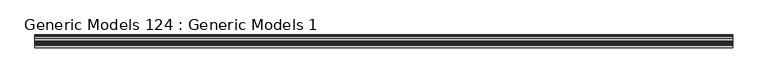
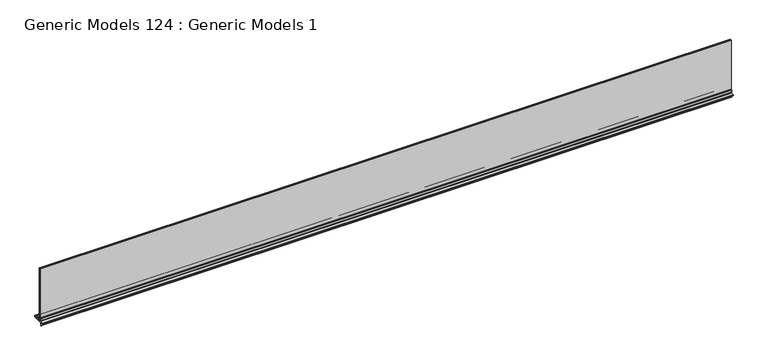
"""IFC4 building model written with IfcOpenShell, lengths in millimetres: proxy geometry, Generic Models 124 : Generic Models 1."""

import ifcopenshell
import ifcopenshell.guid

model = None  # the IFC model being written
_history = None  # IfcOwnerHistory: only IFC2X3 demands one
_inside = {}  # id of a spatial element -> (the spatial element, [elements in it])
_under = {}  # id of a project, library or spatial element -> (it, [spatial elements below it])
_declared = {}  # id of a project -> (the project, [libraries it declares])
_typed = {}  # id of a type object -> (the type object, [elements of that type])
_made_of = {}  # id of a material, layer set ... -> (it, [elements and type objects made of it])


def new_model(schema):
    """Start an empty IFC model of exactly this schema.

    Asked for "IFC4X3", IfcOpenShell would pick the latest addendum, in which some entities
    have other attributes; the version numbers below select the first issue.
    IFC2X3 requires an IfcOwnerHistory on every rooted entity: one is made here for all.
    """
    global model, _history
    if schema == "IFC4X3":
        model = ifcopenshell.file(schema_version=(4, 3, 0, 0))
    else:
        model = ifcopenshell.file(schema=schema)
    _inside.clear()
    _under.clear()
    _declared.clear()
    _typed.clear()
    _made_of.clear()
    _history = None
    if model.schema == "IFC2X3":
        org = make("IfcOrganization", Name="unknown")
        user = make(
            "IfcPersonAndOrganization",
            ThePerson=make("IfcPerson", FamilyName="unknown"),
            TheOrganization=org,
        )
        app = make(
            "IfcApplication",
            ApplicationDeveloper=org,
            Version="unknown",
            ApplicationFullName="unknown",
            ApplicationIdentifier="unknown",
        )
        _history = make(
            "IfcOwnerHistory",
            OwningUser=user,
            OwningApplication=app,
            ChangeAction="ADDED",
            CreationDate=0,
        )
    return model


def make(cls, **values):
    """One entity of the class cls with the attributes given. An attribute that is None is left unset."""
    return model.create_entity(
        cls, **{name: value for name, value in values.items() if value is not None}
    )


def rooted(cls, **values):
    """An entity with a GlobalId (a new one), such as an element, a storey or a relation."""
    return make(cls, GlobalId=ifcopenshell.guid.new(), OwnerHistory=_history, **values)


def si_unit(unit_type, name, prefix=None):
    """IfcSIUnit, for example si_unit("LENGTHUNIT", "METRE", prefix="MILLI")."""
    return make("IfcSIUnit", UnitType=unit_type, Prefix=prefix, Name=name)


def assignment(units):
    """IfcUnitAssignment: the units of a project."""
    return None if units is None else make("IfcUnitAssignment", Units=units)


def point(xyz):
    """IfcCartesianPoint."""
    return None if xyz is None else make("IfcCartesianPoint", Coordinates=xyz)


def direction(xyz):
    """IfcDirection."""
    return None if xyz is None else make("IfcDirection", DirectionRatios=xyz)


def frame(location, z_axis=None, x_axis=None):
    """IfcAxis2Placement3D, a coordinate frame: its origin and axes. An axis left out is left unset."""
    return make(
        "IfcAxis2Placement3D",
        Location=point(location),
        Axis=direction(z_axis),
        RefDirection=direction(x_axis),
    )


def frame_2d(location, x_axis=None):
    """IfcAxis2Placement2D, a coordinate frame in the plane: its origin and x axis."""
    return make(
        "IfcAxis2Placement2D", Location=point(location), RefDirection=direction(x_axis)
    )


def origin():
    """The frame at (0, 0, 0) with its axes left unset."""
    return frame((0.0, 0.0, 0.0))


def place(relative_to, where):
    """IfcLocalPlacement: puts the frame where relative to a parent placement (None: the world)."""
    return make(
        "IfcLocalPlacement", PlacementRelTo=relative_to, RelativePlacement=where
    )


def context(
    kind, dimensions, precision=None, world=None, true_north=None, identifier=None
):
    """IfcGeometricRepresentationContext, for example the 3D "Model" context."""
    return make(
        "IfcGeometricRepresentationContext",
        ContextIdentifier=identifier,
        ContextType=kind,
        CoordinateSpaceDimension=dimensions,
        Precision=precision,
        WorldCoordinateSystem=world,
        TrueNorth=true_north,
    )


def project(units=None, contexts=None):
    """IfcProject with its units and contexts."""
    return rooted(
        "IfcProject",
        Name="project",
        RepresentationContexts=contexts,
        UnitsInContext=assignment(units),
    )


def spatial(cls, under=None, at=None, **own):
    """A site, building, storey or space (cls), placed at a placement, below another one or the project."""
    s = rooted(cls, ObjectPlacement=at, **own)
    if under is not None:
        _under.setdefault(under.id(), (under, []))[1].append(s)
    return s


def polyline(points):
    """IfcPolyline through the points."""
    return make("IfcPolyline", Points=[point(p) for p in points])


def circle_curve(where, radius):
    """IfcCircle in the frame where."""
    return make("IfcCircle", Position=where, Radius=radius)


def trimmed(basis, trim1, trim2, sense, master):
    """IfcTrimmedCurve: the piece of a basis curve between two trims."""
    return make(
        "IfcTrimmedCurve",
        BasisCurve=basis,
        Trim1=trim1,
        Trim2=trim2,
        SenseAgreement=sense,
        MasterRepresentation=master,
    )


def segment(curve, same_sense, transition):
    """IfcCompositeCurveSegment."""
    return make(
        "IfcCompositeCurveSegment",
        Transition=transition,
        SameSense=same_sense,
        ParentCurve=curve,
    )


def composite_curve(segments, self_intersect=None):
    """IfcCompositeCurve: segments joined end to end."""
    return make("IfcCompositeCurve", Segments=segments, SelfIntersect=self_intersect)


def outline(outer, holes=None, kind="AREA"):
    """IfcArbitraryClosedProfileDef: a profile drawn as a closed curve; with holes, ...WithVoids."""
    if holes is None:
        return make("IfcArbitraryClosedProfileDef", ProfileType=kind, OuterCurve=outer)
    return make(
        "IfcArbitraryProfileDefWithVoids",
        ProfileType=kind,
        OuterCurve=outer,
        InnerCurves=holes,
    )


def extrude(swept, where, along, depth):
    """IfcExtrudedAreaSolid: the profile swept, set in the frame where, extruded along a direction by depth."""
    return make(
        "IfcExtrudedAreaSolid",
        SweptArea=swept,
        Position=where,
        ExtrudedDirection=direction(along),
        Depth=depth,
    )


def shape(context_of_items, identifier, shape_type, items):
    """IfcShapeRepresentation: the items that make up one representation, for example the "Body"."""
    return make(
        "IfcShapeRepresentation",
        ContextOfItems=context_of_items,
        RepresentationIdentifier=identifier,
        RepresentationType=shape_type,
        Items=items,
    )


def source(mapping_origin, context_of_items, identifier, shape_type, items):
    """IfcRepresentationMap: a shape defined once, which mapped items show again and again."""
    return make(
        "IfcRepresentationMap",
        MappingOrigin=mapping_origin,
        MappedRepresentation=shape(context_of_items, identifier, shape_type, items),
    )


def transform(
    local_origin,
    x_axis=None,
    y_axis=None,
    z_axis=None,
    scale=None,
    scale2=None,
    scale3=None,
    uniform=True,
):
    """IfcCartesianTransformationOperator3D, or its non-uniform kind. x_axis, y_axis, z_axis: its Axis1, 2, 3."""
    if uniform:
        return make(
            "IfcCartesianTransformationOperator3D",
            Axis1=direction(x_axis),
            Axis2=direction(y_axis),
            LocalOrigin=point(local_origin),
            Scale=scale,
            Axis3=direction(z_axis),
        )
    return make(
        "IfcCartesianTransformationOperator3DnonUniform",
        Axis1=direction(x_axis),
        Axis2=direction(y_axis),
        LocalOrigin=point(local_origin),
        Scale=scale,
        Axis3=direction(z_axis),
        Scale2=scale2,
        Scale3=scale3,
    )


def mapped(mapping_source, mapping_target):
    """IfcMappedItem: shows the shape of a source again, moved by a transform."""
    return make(
        "IfcMappedItem", MappingSource=mapping_source, MappingTarget=mapping_target
    )


def made_of(thing, what):
    """Note that an element or type object is made of a material, layer set ...; save() writes the relation."""
    if what is not None:
        _made_of.setdefault(what.id(), (what, []))[1].append(thing)
    return thing


def element(
    cls,
    number,
    at=None,
    inside=None,
    cuts=None,
    type_object=None,
    material=None,
    context=None,
    identifier="Body",
    shape_type=None,
    held_by="IfcProductDefinitionShape",
    body=None,
    shapes=None,
    **own,
):
    """One element of the class cls, such as IfcWall. Its Tag is "e" and its number.

    at: its placement. inside: the storey or other place that contains it. cuts: it is an
    opening in that element (IfcRelVoidsElement). A single representation is given by context,
    identifier, shape_type and body (its items); several are given by shapes. held_by: the class
    of the entity that holds the representations. save() writes the other relations.
    """
    e = rooted(cls, Tag="e%d" % number, ObjectPlacement=at, **own)
    if body is not None:
        shapes = [shape(context, identifier, shape_type, body)]
    if shapes is not None:
        e.Representation = make(held_by, Representations=shapes)
    if inside is not None:
        _inside.setdefault(inside.id(), (inside, []))[1].append(e)
    if cuts is not None:
        rooted(
            "IfcRelVoidsElement", RelatingBuildingElement=cuts, RelatedOpeningElement=e
        )
    if type_object is not None:
        _typed.setdefault(type_object.id(), (type_object, []))[1].append(e)
    return made_of(e, material)


def aggregate(whole, parts):
    """IfcRelAggregates: a whole, such as a stair, and the parts it consists of."""
    return rooted("IfcRelAggregates", RelatingObject=whole, RelatedObjects=parts)


def save(model, path):
    """Write the relations noted so far, then the file.

    IfcRelAggregates (storeys below a building ...), IfcRelContainedInSpatialStructure (elements
    in a storey), IfcRelDefinesByType, IfcRelAssociatesMaterial and IfcRelDeclares: one each for
    every whole, place, type object, material and project.
    """
    for whole, parts in _under.values():
        aggregate(whole, parts)
    for where, things in _inside.values():
        rooted(
            "IfcRelContainedInSpatialStructure",
            RelatedElements=things,
            RelatingStructure=where,
        )
    for kind, things in _typed.values():
        rooted("IfcRelDefinesByType", RelatedObjects=things, RelatingType=kind)
    for what, things in _made_of.values():
        rooted("IfcRelAssociatesMaterial", RelatedObjects=things, RelatingMaterial=what)
    for by, libraries in _declared.values():
        rooted("IfcRelDeclares", RelatingContext=by, RelatedDefinitions=libraries)
    model.write(path)


def generic_models_124_generic_models_1_1996d743(model_context):
    return source(origin(), model_context, "Body", "SweptSolid", [
        extrude(outline(composite_curve([segment(polyline([(6990.9493503, 124213.5950923), (6972.8808069, 124213.5950923), (6972.8808069, 124216.7700923), (6970.594803, 124216.7700923), (6970.594803, 124213.5950923), (6953.0870538, 124213.5950923), (6953.0870538, 124216.7700923), (6950.8010499, 124216.7700923), (6950.8010499, 124213.5950923), (6933.7739503, 124213.5950923), (6933.7739503, 124215.6778923), (6930.5989503, 124215.6778923), (6930.5989503, 124213.5950923), (6913.4995677, 124213.5950923), (6913.4995677, 124216.7700923), (6911.2135677, 124216.7700923), (6911.2135677, 124213.5950923), (6874.7443999, 124213.5950923), (6874.7443999, 124178.2232047)]), True, "CONTINUOUS"), segment(trimmed(circle_curve(frame_2d((6874.0458997, 124178.2255456)), 0.6985041), [point((6874.7443999, 124178.2232047))], [point((6873.3473999, 124178.2280053))], False, "CARTESIAN"), True, "CONTINUOUS"), segment(polyline([(6873.3473999, 124178.2280053), (6873.3473999, 124213.5950923), (6848.4595655, 124213.5950923), (6848.4595655, 124214.9920923), (6854.8095655, 124214.9920923), (6854.8095655, 124217.2780923), (6846.9059999, 124217.2780923), (6846.9059999, 124226.2095157), (6874.7697999, 124228.6318855), (6909.7201999, 124228.6318855), (6909.7201999, 124233.5086782), (6913.7333271, 124233.5086782), (6913.7333271, 124227.0897386), (6915.7146015, 124227.0897386), (6915.7146015, 124235.0399316), (6924.1219371, 124235.0399316), (6924.1219371, 124235.9797281), (6941.6479371, 124235.9797281), (6941.6479371, 124238.2657281), (6924.1219371, 124238.2657281), (6924.1219371, 124246.9525281), (6921.0739643, 124246.9525281), (6921.0739643, 124250.1275281), (6950.4871883, 124250.1275281), (6950.4871883, 124243.7956956), (6969.5371883, 124243.7956956), (6969.5371883, 124241.4080991), (6971.1373813, 124241.4080991), (6975.0743503, 124238.2330991), (6976.6745433, 124238.2330991), (6976.6745433, 124234.2706956), (6979.8495433, 124234.2706956), (6980.6369953, 124233.4579061), (6990.9493503, 124233.4579061), (6990.9493503, 124223.5264871), (6982.9991573, 124223.5264871), (6982.9991573, 124221.5453095), (6990.9493503, 124221.5453095), (6990.9493503, 124213.5950923)]), True, "CONTINUOUS")], self_intersect=False)), frame((-353.6393476, 0.0, 0.0), z_axis=(1.0, 0.0, 0.0), x_axis=(0.0, 1.0, 0.0)), (0.0, 0.0, 1.0), 7886.7),
        extrude(outline(composite_curve([segment(polyline([(6883.2462578, 124262.4520032), (6884.2693999, 124261.4288611), (6884.2693999, 124257.8482423), (6905.7067708, 124257.8482423), (6903.318482, 124260.2365311), (6903.318482, 124270.1679311), (6915.1461624, 124269.1552811), (6915.1461624, 124266.9929311), (6918.914082, 124266.9929311), (6918.914082, 124259.4491311), (6917.313882, 124259.4491311), (6917.313882, 124257.8482423), (6919.1943999, 124257.8482423), (6919.1943999, 124239.5602423)]), True, "CONTINUOUS"), segment(trimmed(circle_curve(frame_2d((6918.3815999, 124239.5602423)), 0.8128), [point((6919.1943999, 124239.5602423))], [point((6918.3815999, 124238.7474423))], False, "CARTESIAN"), True, "CONTINUOUS"), segment(polyline([(6918.3815999, 124238.7474423), (6905.0465999, 124238.7474423)]), True, "CONTINUOUS"), segment(trimmed(circle_curve(frame_2d((6903.0653999, 124238.7474423)), 1.9812), [point((6905.0465999, 124238.7474423))], [point((6901.0841999, 124238.7474423))], True, "CARTESIAN"), True, "CONTINUOUS"), segment(polyline([(6901.0841999, 124238.7474423), (6888.8921999, 124238.7474423), (6888.8921999, 124233.4388423), (6883.2787999, 124233.4388423), (6883.2787999, 124241.3636423), (6881.3737999, 124241.3636423), (6881.3737999, 124238.0616423), (6879.6973999, 124238.0616423), (6879.6973999, 124236.0296423), (6877.1319999, 124236.0296423)]), True, "CONTINUOUS"), segment(trimmed(circle_curve(frame_2d((6877.1319999, 124238.4172423)), 2.3876), [point((6877.1319999, 124236.0296423))], [point((6874.7443999, 124238.4172423))], False, "CARTESIAN"), True, "CONTINUOUS"), segment(polyline([(6874.7443999, 124238.4172423), (6874.7443999, 124260.7184423), (6877.1319999, 124260.7184423), (6879.6673605, 124268.5242658), (6882.1103999, 124268.7138161), (6882.1103999, 124266.6874423), (6883.2462578, 124266.6874423), (6883.2462578, 124262.4520032)]), True, "CONTINUOUS")], self_intersect=False)), frame((-353.6393476, 0.0, 0.0), z_axis=(1.0, 0.0, 0.0), x_axis=(0.0, 1.0, 0.0)), (0.0, 0.0, 1.0), 7886.7),
        extrude(outline(polyline([(7533.0606524, 6902.524732), (7533.0606524, 6897.762232), (-353.6393476, 6897.762232), (-353.6393476, 6902.524732), (7533.0606524, 6902.524732)])), frame((0.0, 0.0, 124258.6419923), z_axis=(0.0, 0.0, 1.0), x_axis=(1.0, 0.0, 0.0)), (0.0, 0.0, 1.0), 602.3375481),
        extrude(outline(polyline([(7533.0606524, 6896.968482), (7533.0606524, 6890.6193999), (-353.6393476, 6890.6193999), (-353.6393476, 6896.968482), (7533.0606524, 6896.968482)])), frame((0.0, 0.0, 124258.6419923), z_axis=(0.0, 0.0, 1.0), x_axis=(1.0, 0.0, 0.0)), (0.0, 0.0, 1.0), 6.35),
        extrude(outline(polyline([(7533.0606524, 6889.8256499), (7533.0606524, 6885.0631499), (-353.6393476, 6885.0631499), (-353.6393476, 6889.8256499), (7533.0606524, 6889.8256499)])), frame((0.0, 0.0, 124258.6419923), z_axis=(0.0, 0.0, 1.0), x_axis=(1.0, 0.0, 0.0)), (0.0, 0.0, 1.0), 602.3375481),
    ])


if __name__ == "__main__":
    model = new_model("IFC4")
    model_context = context("Model", 3, world=origin())
    ifc_project = project(units=[si_unit("LENGTHUNIT", "METRE", prefix="MILLI")], contexts=[model_context])
    site = spatial("IfcSite", under=ifc_project)
    building = spatial("IfcBuilding", under=site)
    placement = place(None, origin())
    generic_models_124_generic_models_1_shape = generic_models_124_generic_models_1_1996d743(model_context)
    element("IfcBuildingElementProxy", 1, Name="Generic Models 124 : Generic Models 1", ObjectType="Generic Models 124 : Generic Models 1", at=placement, inside=building, context=model_context, shape_type="MappedRepresentation", body=[
        mapped(generic_models_124_generic_models_1_shape, transform((0.0, 0.0, 0.0), x_axis=(1.0, 0.0, 0.0), y_axis=(0.0, 1.0, 0.0), z_axis=(0.0, 0.0, 1.0))),
    ])
    save(model, "model.ifc")

# Revit data of these elements
# Element 1 (IfcBuildingElementProxy, "Generic Models 124 : Generic Models 1")
#   Materials on its faces: "_WINDOW PER SCHEDULE"
# Materials
#   "_WINDOW PER SCHEDULE": class "Generic", colour RGB 255 255 255, transparency 0, Cost = 0
